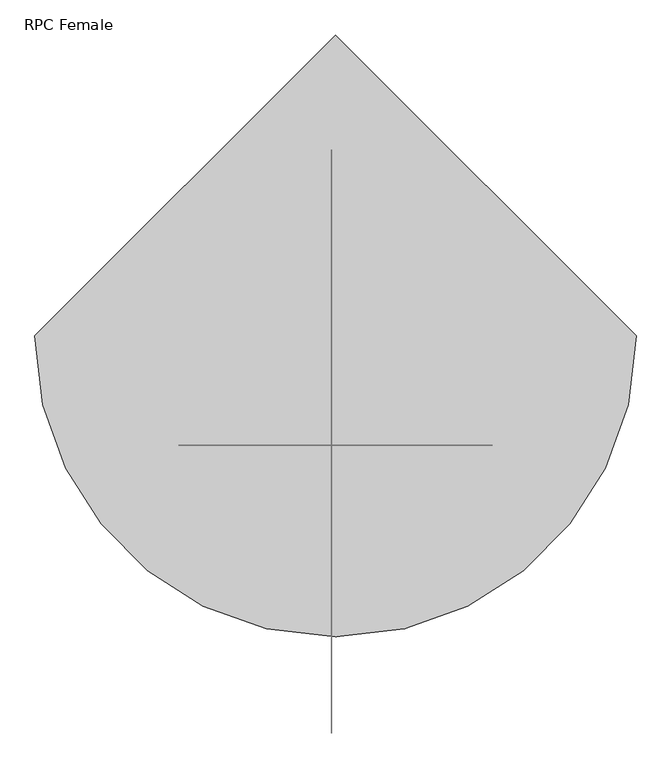
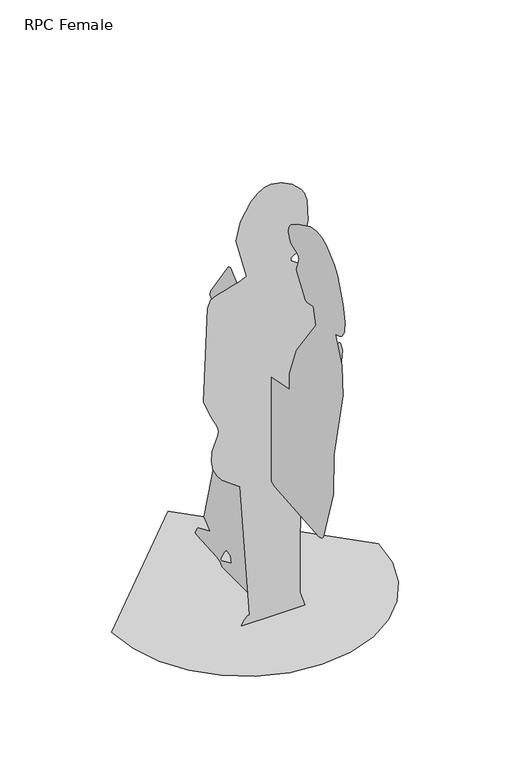
"""IFC4 building model written with IfcOpenShell, lengths in millimetres: proxy geometry, RPC Female : Cynthia."""

from ifc_helpers import new_model, si_unit, origin, place, context, project, spatial, triangles, source, transform, mapped, element, save


def rpc_female_c3b5a3e1(model_context):
    return source(origin(), model_context, "Body", "Tessellation", [
        triangles([(-437.3060472, 0.0, 2.93e-05), (-425.7451249, -100.2016327, 2.93e-05), (-392.8196637, -192.220807, 2.93e-05), (-341.1660942, -273.421065, 2.93e-05), (-273.4210832, -341.1661669, 2.93e-05), (-192.2207525, -392.8196274, 2.93e-05), (-100.2015873, -425.7450522, 2.93e-05), (1.91e-05, -437.3060472, 2.93e-05), (100.2016418, -425.7451249, 2.93e-05), (192.2208252, -392.8196637, 2.93e-05), (273.4210832, -341.1660942, 2.93e-05), (341.1662395, -273.4210832, 2.93e-05), (392.8196274, -192.2207344, 2.93e-05), (425.7450522, -100.2015691, 2.93e-05), (437.3060472, 3.36e-05, 2.93e-05), (-5.73e-05, 437.3060835, 2.93e-05), (-5.5814595, 72.2469164, 69.4963894), (-5.5814595, 67.0311828, 46.0256926), (-5.5814618, 124.4040072, 19.9471473), (-5.5814618, 129.6197135, 25.1628355), (-5.5814606, 107.6002908, 62.2269748), (-5.5814595, 95.7176132, 74.7120821), (-5.5814595, -28.6037251, 4.4e-06), (-5.5814589, -39.8908927, 35.5942709), (-5.5814589, -42.4985824, 37.2668455), (-5.5814583, -45.6386024, 39.1828236), (-5.5814583, -48.9915681, 41.1595925), (-5.5814583, -52.2381586, 43.0148617), (-5.5814583, -55.0589485, 44.5657618), (-5.5814583, -57.1346439, 45.630268), (-5.5814583, -58.1458422, 46.0256972), (-5.5814595, -58.1459239, 5.3e-06), (-5.5814589, -108.9534877, 6.8e-06), (-5.5814578, -116.5758876, 29.8220396), (-5.5814544, -109.3237594, 163.617066), (-5.5814447, -45.4571863, 488.7460396), (-5.5814447, -47.7144613, 510.22398), (-5.5814447, -52.930154, 512.8317787), (-5.5814442, -176.693648, 461.1355883), (-5.5814407, -431.0103195, 441.4519423), (-5.5814407, -446.7163739, 445.0275962), (-5.5814402, -456.1588572, 455.8254473), (-5.5814334, -511.6812675, 636.0533998), (-5.5814294, -514.5206291, 776.2252218), (-5.581422, -566.7675127, 1012.4535353), (-5.5814192, -561.4620226, 1112.6385538), (-5.5814163, -522.3441341, 1198.6978357), (-5.5814163, -544.766203, 1204.597403), (-5.5814158, -561.2101121, 1214.9823069), (-5.5814152, -573.9146782, 1236.2579704), (-5.5814135, -577.4590839, 1272.8749214), (-5.5814124, -566.4222939, 1329.2833969), (-5.5814107, -535.3834182, 1409.9341427), (-5.5814101, -516.7875329, 1433.7646648), (-5.5814095, -472.5757693, 1474.3213463), (-5.5814095, -445.9834971, 1486.7823589), (-5.5814101, -415.7492961, 1491.1889214), (-5.5814107, -381.3848602, 1485.4078789), (-5.5814124, -308.1104447, 1450.1712215), (-5.5814135, -271.6909563, 1426.3745636), (-5.5814141, -259.9824413, 1410.5522736), (-5.5814152, -256.5010404, 1391.3537361), (-5.5814158, -264.1664701, 1368.2083466), (-5.5814158, -270.5527808, 1361.5173306), (-5.5814158, -307.4895524, 1345.9739479), (-5.5814158, -313.689719, 1341.0972107), (-5.5814158, -316.3235335, 1334.3062008), (-5.5814163, -314.5106718, 1321.5905525), (-5.5814175, -303.2843222, 1289.972715), (-5.5814175, -303.9330653, 1281.3193188), (-5.5814186, -344.8554039, 1227.4574902), (-5.5814192, -350.225752, 1216.9527534), (-5.5814192, -354.0102593, 1213.1380154), (-5.5814192, -360.9106739, 1211.8318451), (-5.581418, -397.1671454, 1216.9527534), (-5.5814197, -412.8142282, 1162.1877823), (-5.5814254, -300.7219422, 1007.465613), (-5.5814294, -262.9223781, 903.7025425), (-5.5814311, -261.5586532, 849.245256), (-5.5814334, -151.2455011, 828.1027239), (-5.5814334, -131.1658673, 828.382358), (-5.5814322, -146.9134072, 873.4852736), (-5.5814322, -146.8129955, 875.3236788), (-5.5814322, -136.528476, 880.5995195), (-5.5814294, 66.2908937, 1062.7625284), (-5.5814294, 72.9542315, 1068.1179428), (-5.58143, 85.3176393, 1063.7725685), (-5.5814356, 186.9121194, 916.7362673), (-5.5814362, 189.6004001, 904.0100819), (-5.5814373, 74.8547605, 802.3037899), (-5.5814385, 53.5232047, 768.5295433), (-5.5814385, 40.9526375, 757.9702314), (-5.5814385, 7.0502453, 750.1467264), (-5.5814396, -30.7395867, 681.3431499), (-5.5814396, -32.0672991, 677.1266922), (-5.5814402, -2.7970188, 673.1422697), (-5.5814413, 74.8547605, 666.6952068), (-5.5814606, 223.5024732, 113.8299342), (-5.5814606, 192.3028696, 86.4272827), (-5.5814606, 189.6004001, 82.5356507), (-5.5814629, 257.4046916, 53.8492703), (-5.5814629, 261.0574302, 50.6335736), (-5.5814635, 266.9933869, 41.9573681), (-5.5814635, 270.402463, 33.1798516), (-5.5814635, 270.8967278, 29.8373366), (-5.5814635, 270.4438667, 27.7706795), (-5.5814635, 262.2121017, 24.672413), (-5.5814623, 148.399036, 17.7234889), (-5.5814623, 129.6197135, 12.1235673), (-5.5814623, 119.228015, 0.0), (-103.2161744, -158.8626324, 3.1383159), (-93.5649829, -158.8626324, 19.2429933), (-88.6212531, -158.8626324, 24.4594445), (-82.9718341, -158.8626324, 28.4095327), (-76.7114059, -158.8626324, 30.3785123), (-108.0056803, -158.8626688, 484.1452303), (-166.5179246, -158.8626688, 527.9972775), (-183.6323596, -158.8626688, 549.7335234), (-196.1560501, -158.8626688, 575.2326937), (-202.051348, -158.8626688, 604.6170193), (-199.2806414, -158.8626688, 638.0087311), (-180.7338447, -158.8626688, 688.9253906), (-179.5105545, -158.8626688, 700.1741953), (-181.0256691, -158.8626688, 711.0286926), (-186.0299967, -158.8626688, 724.8032879), (-192.7432497, -158.8626688, 739.7140783), (-208.556347, -158.8626688, 771.7153954), (-227.9670263, -158.8626688, 820.5585623), (-215.5927998, -158.8627051, 1139.719677), (-204.4963295, -158.8627051, 1164.795472), (-195.7042972, -158.8627051, 1170.2251551), (-178.3999392, -158.8627051, 1176.5906822), (-156.0961225, -158.8627051, 1183.4371393), (-132.3056233, -158.8627051, 1190.3085222), (-110.5413813, -158.8627051, 1196.7500622), (-94.3161544, -158.8627051, 1202.3061911), (-87.1428368, -158.8627051, 1206.5211954), (-121.0449553, -158.8627051, 1339.5217255), (-105.9598841, -158.8627233, 1402.4776211), (-72.2006802, -158.8627233, 1459.3937691), (-51.1399244, -158.8627233, 1480.6096252), (-28.7965753, -158.8627233, 1494.3423626), (-6.2993163, -158.8627233, 1498.6009689), (28.3786116, -158.8627233, 1491.3014145), (62.9444138, -158.8627233, 1473.3404469), (92.2084978, -158.8627233, 1445.5319698), (103.2306357, -158.8627233, 1428.1888424), (112.1217082, -158.8627233, 1400.9906479), (114.2135863, -158.8627051, 1329.2272957), (96.1615087, -158.8627051, 1258.9099308), (79.8726138, -158.8627051, 1233.5191841), (58.8970909, -158.8627051, 1219.5604431), (58.8970909, -158.8627051, 1209.1289577), (105.4403209, -158.8627051, 1177.1577988), (186.6819918, -158.8627051, 1146.5404089), (190.9102947, -158.8627051, 1130.2535397), (197.4606216, -158.8627051, 874.561952), (217.1153449, -158.8627051, 870.6129925), (219.4355885, -158.8627051, 869.5271576), (221.3550207, -158.8627051, 866.9867603), (227.9670444, -158.8626688, 839.7671282), (217.976248, -158.8626688, 726.675848), (216.7788284, -158.8626688, 725.5374001), (198.4189752, -158.8626688, 721.3537165), (197.1134226, -158.8626688, 721.4601053), (188.2935758, -158.8626688, 736.0854481), (176.2505791, -158.8626688, 750.1465811), (172.5435924, -158.8626688, 744.3788372), (169.4577161, -158.8626688, 737.624235), (166.7655839, -158.8626688, 730.2871828), (164.2398296, -158.8626688, 722.7722345), (161.6531779, -158.8626688, 715.4839439), (158.7782626, -158.8626688, 708.8267195), (155.3877173, -158.8626688, 703.2051149), (164.598892, -158.8626688, 582.3868355), (159.7289131, -158.8626688, 557.9940293), (150.1720292, -158.8626688, 536.3024028), (143.4522449, -158.8626688, 528.6089407), (105.4337806, -158.8626688, 509.5450607), (96.8766176, -158.8626688, 503.2558007), (90.1913244, -158.8626688, 494.5766793), (88.7456459, -158.8626324, 49.410397), (105.4366693, -158.8626324, 7.4e-05), (-104.3910663, -158.8626324, 7.4e-05)], [[15, 16, 1], [14, 15, 1], [14, 1, 2], [13, 14, 2], [13, 2, 3], [13, 3, 4], [12, 13, 4], [11, 12, 4], [11, 4, 5], [11, 5, 6], [11, 6, 7], [11, 7, 8], [11, 8, 9], [11, 9, 10], [23, 17, 18], [110, 23, 18], [110, 18, 19], [109, 110, 19], [17, 23, 24], [31, 32, 33], [31, 33, 34], [109, 19, 20], [108, 109, 20], [88, 89, 90], [82, 83, 84], [85, 86, 87], [105, 106, 107], [104, 105, 107], [103, 104, 107], [102, 103, 107], [101, 102, 107], [100, 101, 107], [100, 107, 108], [100, 108, 20], [100, 20, 21], [100, 21, 22], [87, 88, 90], [85, 87, 90], [84, 85, 90], [84, 90, 91], [84, 91, 92], [84, 92, 93], [82, 84, 93], [81, 82, 93], [81, 93, 94], [80, 81, 94], [80, 94, 95], [99, 100, 22], [17, 24, 25], [17, 25, 26], [31, 34, 35], [30, 31, 35], [17, 26, 27], [17, 27, 28], [17, 28, 29], [29, 30, 35], [17, 29, 35], [22, 17, 35], [99, 22, 35], [98, 99, 35], [97, 98, 35], [97, 35, 36], [97, 36, 37], [96, 97, 37], [96, 37, 38], [95, 96, 38], [80, 95, 38], [80, 38, 39], [79, 80, 39], [79, 39, 40], [79, 40, 41], [79, 41, 42], [79, 42, 43], [79, 43, 44], [78, 79, 44], [77, 78, 44], [77, 44, 45], [77, 45, 46], [76, 77, 46], [76, 46, 47], [75, 76, 47], [72, 73, 74], [71, 72, 74], [61, 62, 63], [60, 61, 63], [60, 63, 64], [59, 60, 64], [59, 64, 65], [59, 65, 66], [58, 59, 66], [57, 58, 66], [56, 57, 66], [55, 56, 66], [54, 55, 66], [54, 66, 67], [53, 54, 67], [52, 53, 67], [52, 67, 68], [51, 52, 68], [50, 51, 68], [49, 50, 68], [48, 49, 68], [47, 48, 68], [75, 47, 68], [74, 75, 68], [71, 74, 68], [70, 71, 68], [69, 70, 68], [183, 184, 111], [183, 111, 112], [183, 112, 113], [183, 113, 114], [183, 114, 115], [182, 183, 115], [181, 182, 115], [181, 115, 116], [154, 155, 156], [164, 165, 166], [180, 181, 116], [163, 164, 166], [162, 163, 166], [162, 166, 167], [161, 162, 167], [160, 161, 167], [159, 160, 167], [158, 159, 167], [157, 158, 167], [180, 116, 117], [180, 117, 118], [180, 118, 119], [180, 119, 120], [180, 120, 121], [180, 121, 122], [179, 180, 122], [179, 122, 123], [178, 179, 123], [177, 178, 123], [176, 177, 123], [175, 176, 123], [174, 175, 123], [174, 123, 124], [174, 124, 125], [173, 174, 125], [172, 173, 125], [171, 172, 125], [170, 171, 125], [169, 170, 125], [169, 125, 126], [168, 169, 126], [168, 126, 127], [167, 168, 127], [157, 167, 127], [157, 127, 128], [156, 157, 128], [154, 156, 128], [153, 154, 128], [153, 128, 129], [153, 129, 130], [153, 130, 131], [153, 131, 132], [153, 132, 133], [153, 133, 134], [153, 134, 135], [153, 135, 136], [153, 136, 137], [152, 153, 137], [151, 152, 137], [150, 151, 137], [149, 150, 137], [149, 137, 138], [149, 138, 139], [148, 149, 139], [147, 148, 139], [146, 147, 139], [146, 139, 140], [145, 146, 140], [145, 140, 141], [144, 145, 141], [144, 141, 142], [144, 142, 143]], closed=False),
    ])


if __name__ == "__main__":
    model = new_model("IFC4")
    model_context = context("Model", 3, world=origin())
    ifc_project = project(units=[si_unit("LENGTHUNIT", "METRE", prefix="MILLI")], contexts=[model_context])
    site = spatial("IfcSite", under=ifc_project)
    building = spatial("IfcBuilding", under=site)
    placement = place(None, origin())
    rpc_female_shape = rpc_female_c3b5a3e1(model_context)
    element("IfcBuildingElementProxy", 1, Name="RPC Female : Cynthia", ObjectType="RPC Female : Cynthia", at=placement, inside=building, context=model_context, shape_type="MappedRepresentation", body=[
        mapped(rpc_female_shape, transform((0.0, 0.0, 0.0), x_axis=(1.0, 0.0, 0.0), y_axis=(0.0, 1.0, 0.0), z_axis=(0.0, 0.0, 1.0))),
    ])
    save(model, "model.ifc")

# Revit data of these elements
# Type "RPC Female : Cynthia"
#   built-in parameter 1005198 = "{2, 15},{22, RPC-8-FXA2-QQQ0-UGV2-6},{1, 0},{1, 0},{2, 15},{1, 8},{5, Color},{1, 0},{1, 0},{3, 0.8},{3, 0.8},{3, 0.8},{1, 8},{7, BBoxMin},{1, 0},{1, 0},{1, 0},{1, 0},{1, 0},{1, 8},{7, BBoxMax},{1, 0},{1, 0},{1, 0},{1, 0},{1, 0},{2, 11},{9, RPCTypeId},{1, 0},{1, 0},{22, RPC-8-FXA2-QQQ0-UGV2-6},{1, 6},{14, RPCPlantHeight},{1, 0},{1, 0},{7, 4.91667},{2, 11},{7, keyword},{1, 0},{1, 0},{43, :RPCs:People [Seated-Business]:Geometry:RPC},{2, 11},{8, category},{1, 0},{1, 0},{24, People [Seated-Business]},{2, 11},{12, LocalizedUID},{1, 0},{1, 0},{7, Cynthia},{2, 14},{6, Height},{1, 0},{1, 0},{7, 4.91667},{1, 2},{16, Cast Reflections},{1, 0},{1, 0},{1, 0},{1, 2},{6, Jitter},{1, 0},{1, 0},{1, 1},{1, 2},{9, Billboard},{1, 0},{1, 0},{1, 0},{1, 2},{12, Cast Shadows},{1, 0},{1, 0},{1, 1},{1, 2},{20, Apply Filter Effects},{1, 0},{1, 0},{1, 0},{2, 11},{28, Apply Filter Effects-Text-FC},{1, 0},{1, 0},{4, None},{21, assetlibrary_base.fbx},{1, 5},"
#   built-in parameter 1005195 = "RPC-8-FXA2-QQQ0-UGV2-6"
#   Height = 0
